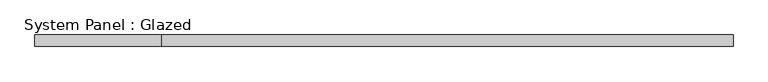
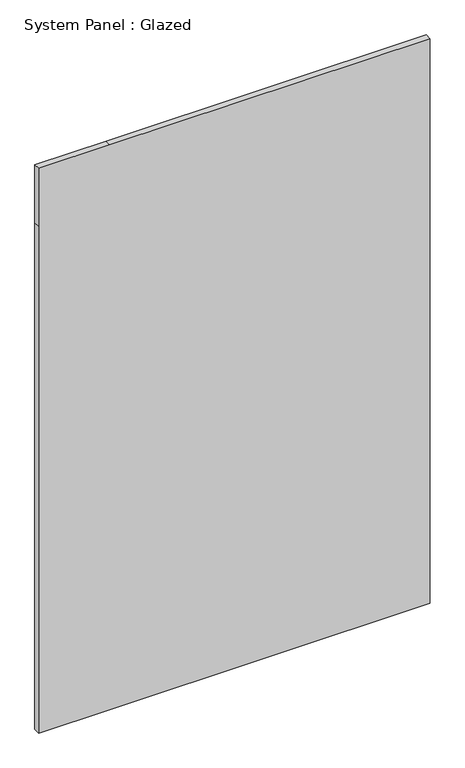
"""IFC4 building model written with IfcOpenShell, lengths in millimetres: plate geometry, System Panel : Glazed."""

from ifc_helpers import new_model, si_unit, frame, origin, place, context, project, spatial, polyline, outline, extrude, source, transform, mapped, element, save


def system_panel_glazed_bb2f95a6(model_context):
    return source(origin(), model_context, "Body", "SweptSolid", [
        extrude(outline(polyline([(0.0, -768.35), (0.0, -488.95), (0.0, 768.35), (2101.85, 768.35), (2343.15, 768.35), (2343.15, -488.95), (2343.15, -768.35), (2101.85, -768.35), (0.0, -768.35)])), frame((0.0, -44.45, 0.0), z_axis=(0.0, 1.0, 0.0), x_axis=(0.0, 0.0, 1.0)), (0.0, 0.0, 1.0), 25.4),
    ])


if __name__ == "__main__":
    model = new_model("IFC4")
    model_context = context("Model", 3, world=origin())
    ifc_project = project(units=[si_unit("LENGTHUNIT", "METRE", prefix="MILLI")], contexts=[model_context])
    site = spatial("IfcSite", under=ifc_project)
    building = spatial("IfcBuilding", under=site)
    placement = place(None, origin())
    system_panel_glazed_shape = system_panel_glazed_bb2f95a6(model_context)
    element("IfcPlate", 1, ObjectType="System Panel : Glazed", at=placement, inside=building, context=model_context, shape_type="MappedRepresentation", body=[
        mapped(system_panel_glazed_shape, transform((0.0, 0.0, 0.0), x_axis=(1.0, 0.0, 0.0), y_axis=(0.0, 1.0, 0.0), z_axis=(0.0, 0.0, 1.0))),
    ])
    save(model, "model.ifc")

# Revit data of these elements
# Element 1 (IfcPlate, "System Panel : Glazed")
#   Materials on its faces: "Glass"
# Materials
#   "Glass": class "Glass", colour RGB 0 128 192, transparency 0.75, Cost = 0
